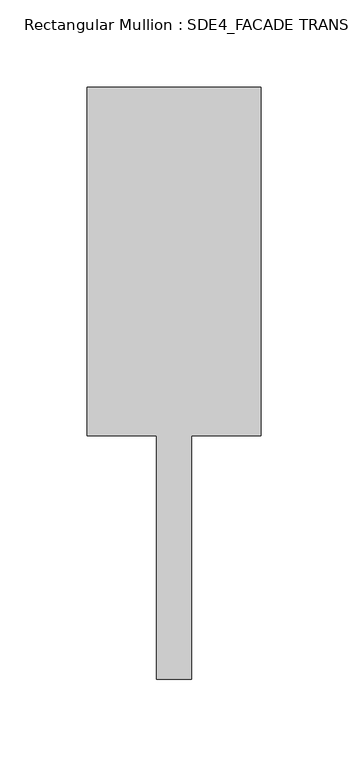
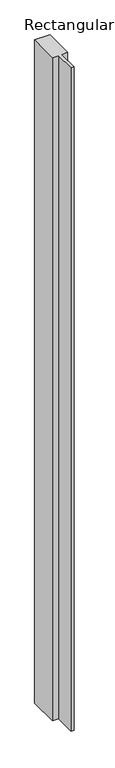
"""IFC4 building model written with IfcOpenShell, lengths in millimetres: member geometry, Rectangular Mullion : SDE4_FACADE TRANSOM TYPE 1."""

from ifc_helpers import new_model, si_unit, frame, origin, place, context, project, spatial, polyline, outline, extrude, source, transform, mapped, element, save


def rectangular_mullion_sde4_facade_transom_type_1_8090ca5d(model_context):
    return source(origin(), model_context, "Body", "SweptSolid", [
        extrude(outline(polyline([(50.0, 132.5), (50.0, -67.5), (10.0, -67.5), (10.0, -207.5), (-10.0, -207.5), (-10.0, -67.5), (-50.0, -67.5), (-50.0, 132.5), (50.0, 132.5)])), frame((0.0, 0.0, -4577.0), z_axis=(0.0, 0.0, 1.0), x_axis=(1.0, 0.0, 0.0)), (0.0, 0.0, 1.0), 4577.0),
    ])


if __name__ == "__main__":
    model = new_model("IFC4")
    model_context = context("Model", 3, world=origin())
    ifc_project = project(units=[si_unit("LENGTHUNIT", "METRE", prefix="MILLI")], contexts=[model_context])
    site = spatial("IfcSite", under=ifc_project)
    building = spatial("IfcBuilding", under=site)
    placement = place(None, origin())
    rectangular_mullion_sde4_facade_transom_type_1_shape = rectangular_mullion_sde4_facade_transom_type_1_8090ca5d(model_context)
    element("IfcMember", 1, ObjectType="Rectangular Mullion : SDE4_FACADE TRANSOM TYPE 1", at=placement, inside=building, context=model_context, shape_type="MappedRepresentation", body=[
        mapped(rectangular_mullion_sde4_facade_transom_type_1_shape, transform((0.0, 0.0, 0.0), x_axis=(1.0, 0.0, 0.0), y_axis=(0.0, 1.0, 0.0), z_axis=(0.0, 0.0, 1.0))),
    ])
    save(model, "model.ifc")

# Revit data of these elements
# Type "Rectangular Mullion : SDE4_FACADE TRANSOM TYPE 1"
#   built-in parameter 1007322 = 1.11549 (stored number, unit not read)
#   built-in parameter 1007321 = 0.164042 (stored number, unit not read)
#   built-in parameter 1007320 = 0.164042 (stored number, unit not read)
